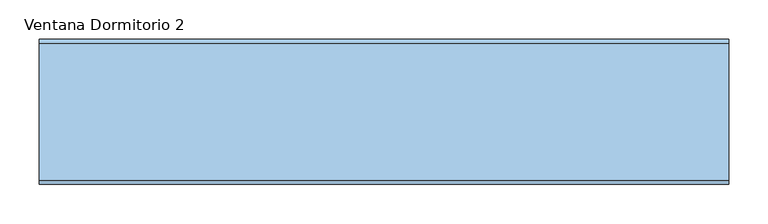
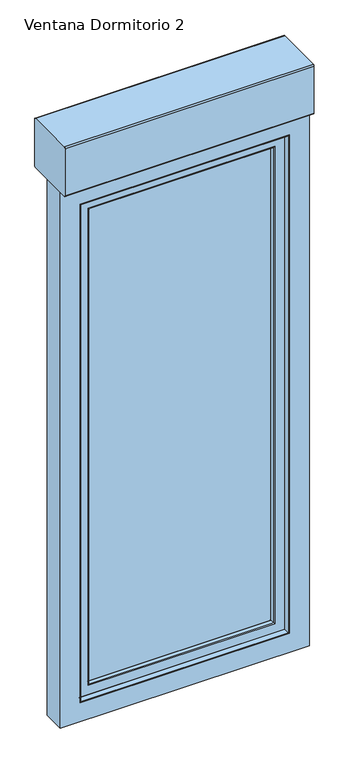
"""IFC4 building model written with IfcOpenShell, lengths in millimetres: window geometry, 2019_ES_Ventana_Replus_re80pvc301_10100_box_1-Hoja_con-Compacto : Ventana Dormitorio 2."""

from ifc_helpers import new_model, si_unit, point, frame, frame_2d, origin, place, context, project, spatial, polyline, circle_curve, ellipse_curve, trimmed, segment, composite_curve, outline, extrude, source, transform, mapped, element, save
from ifc_brep_helpers import plane_surface, cylinder_surface, advanced_brep


def ventana_dormitorio_2_c32e29da(model_context):
    return source(origin(), model_context, "Body", "SolidModel", [
        extrude(outline(composite_curve([segment(trimmed(circle_curve(frame_2d((-55.0, 2815.0)), 5.0), [point((-55.0, 2810.0))], [point((-60.0, 2815.0))], False, "CARTESIAN"), True, "CONTINUOUS"), segment(polyline([(-60.0, 2815.0), (-60.0, 2990.0)]), True, "CONTINUOUS"), segment(trimmed(circle_curve(frame_2d((-55.0, 2990.0)), 5.0), [point((-60.0, 2990.0))], [point((-55.0, 2995.0))], False, "CARTESIAN"), True, "CONTINUOUS"), segment(polyline([(-55.0, 2995.0), (120.0, 2995.0)]), True, "CONTINUOUS"), segment(trimmed(circle_curve(frame_2d((120.0, 2990.0)), 5.0), [point((120.0, 2995.0))], [point((125.0, 2990.0))], False, "CARTESIAN"), True, "CONTINUOUS"), segment(polyline([(125.0, 2990.0), (125.0, 2815.0)]), True, "CONTINUOUS"), segment(trimmed(circle_curve(frame_2d((120.0, 2815.0)), 5.0), [point((125.0, 2815.0))], [point((120.0, 2810.0))], False, "CARTESIAN"), True, "CONTINUOUS"), segment(polyline([(120.0, 2810.0), (-55.0, 2810.0)]), True, "CONTINUOUS")], self_intersect=False)), frame((-440.0, 0.0, 0.0), z_axis=(1.0, 0.0, 0.0), x_axis=(0.0, 1.0, 0.0)), (0.0, 0.0, 1.0), 880.0),
        extrude(outline(polyline([(78.4999991, 1470.0), (118.4999991, 1470.0), (118.4999991, 1360.0), (98.4999991, 1360.0), (98.4999991, 1450.0), (78.4999991, 1450.0), (78.4999991, 1470.0)])), frame((-374.1999993, 0.0, 0.0), z_axis=(1.0, 0.0, 0.0), x_axis=(0.0, 1.0, 0.0)), (0.0, 0.0, 1.0), 12.0),
        extrude(outline(polyline([(-353.9687607, 78.4999991), (-353.9687607, 68.4999991), (-382.4312378, 68.4999991), (-382.4312378, 78.4999991), (-353.9687607, 78.4999991)])), frame((0.0, 0.0, 1435.217127), z_axis=(0.0, 0.0, 1.0), x_axis=(1.0, 0.0, 0.0)), (0.0, 0.0, 1.0), 49.565746),
        extrude(outline(polyline([(909.8, 337.1999993), (2707.2, 337.1999993), (2707.2, -337.1999993), (909.8, -337.1999993), (909.8, 337.1999993)]), holes=[polyline([(2699.2, 329.1999993), (917.8, 329.1999993), (917.8, -329.1999993), (2699.2, -329.1999993), (2699.2, 329.1999993)])]), frame((0.0, 10.9999999, 0.0), z_axis=(0.0, 1.0, 0.0), x_axis=(0.0, 0.0, 1.0)), (0.0, 0.0, 1.0), 16.0),
        extrude(outline(polyline([(909.8131934, 337.1868058), (2707.1868066, 337.1868058), (2707.1868066, -337.1868058), (909.8131934, -337.1868058), (909.8131934, 337.1868058)]), holes=[polyline([(2699.2, 329.1999993), (917.8, 329.1999993), (917.8, -329.1999993), (2699.2, -329.1999993), (2699.2, 329.1999993)])]), frame((0.0, 31.0000001, 0.0), z_axis=(0.0, 1.0, 0.0), x_axis=(0.0, 0.0, 1.0)), (0.0, 0.0, 1.0), 16.0),
        extrude(outline(polyline([(337.1999993, 6.9999997), (-337.1999993, 6.9999997), (-337.1999993, 10.9999999), (337.1999993, 10.9999999), (337.1999993, 6.9999997)])), frame((0.0, 0.0, 903.7946451), z_axis=(0.0, 0.0, 1.0), x_axis=(1.0, 0.0, 0.0)), (0.0, 0.0, 1.0), 1809.4053549),
        extrude(outline(polyline([(337.1999993, 26.9999999), (-337.1999993, 26.9999999), (-337.1999993, 31.0000001), (337.1999993, 31.0000001), (337.1999993, 26.9999999)])), frame((0.0, 0.0, 903.7946451), z_axis=(0.0, 0.0, 1.0), x_axis=(1.0, 0.0, 0.0)), (0.0, 0.0, 1.0), 1809.4053549),
        extrude(outline(polyline([(337.1999993, 47.0000001), (-337.1999993, 47.0000001), (-337.1999993, 51.0000003), (337.1999993, 51.0000003), (337.1999993, 47.0000001)])), frame((0.0, 0.0, 903.7946451), z_axis=(0.0, 0.0, 1.0), x_axis=(1.0, 0.0, 0.0)), (0.0, 0.0, 1.0), 1809.4053549),
        advanced_brep(
        [(327.2913171, -9.2764571, 2697.2913178), (327.2913171, -9.2764571, 922.7086822), (330.1890946, -11.5, 919.8109047), (330.1890946, -11.5, 2700.1890953), (370.1999993, -11.5, 879.8), (370.1999993, -11.5, 2740.2), (-370.1999993, -11.5, 2740.2), (-370.1999993, -11.5, 879.8), (-330.1890946, -11.5, 919.8109047), (-330.1890946, -11.5, 2700.1890953), (-327.2913171, -9.2764571, 922.7086822), (324.1757968, 2.3508228, 2694.1757976), (324.1757968, 2.3508228, 925.8242024), (-324.1757968, 2.3508228, 925.8242024), (324.6739305, 3.0000033, 2694.6739313), (324.6739305, 3.0000033, 925.3260687), (-324.6739305, 3.0000033, 925.3260687), (331.1999993, 3.0000033, 2701.2), (331.1999993, 3.0000033, 918.8), (-331.1999993, 3.0000033, 918.8), (-331.1999993, 3.0000033, 2701.2), (-324.6739305, 3.0000033, 2694.6739313), (331.1999993, 6.9999997, 2701.2), (331.1999993, 6.9999997, 918.8), (-331.1999993, 6.9999997, 918.8), (351.8162192, 6.9999997, 2721.8162199), (351.8162192, 6.9999997, 898.1837801), (-351.8162192, 6.9999997, 898.1837801), (-351.8162192, 6.9999997, 2721.8162199), (-331.1999993, 6.9999997, 2701.2), (349.1999993, 25.6153717, 2719.2), (349.1999993, 25.6153717, 900.8), (-349.1999993, 25.6153717, 900.8), (349.1999993, 56.4999995, 2719.2), (349.1999993, 56.4999995, 900.8), (-349.1999993, 56.4999995, 900.8), (-349.1999993, 56.4999995, 2719.2), (337.1999993, 56.4999995, 2707.2), (337.1999993, 56.4999995, 912.8), (-337.1999993, 56.4999995, 912.8), (-337.1999993, 56.4999995, 2707.2), (337.1999993, 51.0000003, 2707.2), (337.1999993, 51.0000003, 912.8), (-337.1999993, 51.0000003, 912.8), (-337.1999993, 51.0000003, 2707.2), (326.007687, 51.0000003, 2696.0076877), (326.007687, 51.0000003, 923.9923123), (-326.007687, 51.0000003, 923.9923123), (-326.007687, 51.0000003, 2696.0076877), (325.4940999, 51.6693201, 2695.4941006), (325.4940999, 51.6693201, 924.5058994), (-325.4940999, 51.6693201, 924.5058994), (328.8993918, 64.3780426, 2698.8993925), (328.8993918, 64.3780426, 921.1006075), (-328.8993918, 64.3780426, 921.1006075), (332.6234971, 67.3403297, 2702.6234978), (332.6234971, 67.3403297, 917.3765022), (-332.6234971, 67.3403297, 917.3765022), (345.6488427, 67.7951848, 2715.6488434), (345.6488427, 67.7951848, 904.3511566), (-345.6488427, 67.7951848, 904.3511566), (346.1999993, 67.2629391, 2716.2), (346.1999993, 67.2629391, 903.8), (-346.1999993, 67.2629391, 903.8), (347.4370593, 68.4999991, 2717.43706), (347.4370593, 68.4999991, 902.56294), (-347.4370593, 68.4999991, 902.56294), (400.1999993, 68.4999991, 2770.2), (400.1999993, 68.4999991, 849.8), (-400.1999993, 68.4999991, 849.8), (-400.1999993, 68.4999991, 2770.2), (-347.4370593, 68.4999991, 2717.43706), (403.1999993, 65.4999991, 2773.2), (403.1999993, 65.4999991, 846.8), (-403.1999993, 65.4999991, 846.8), (403.1999993, 50.0, 2773.2), (403.1999993, 50.0, 846.8), (-403.1999993, 50.0, 846.8), (-403.1999993, 50.0, 2773.2), (383.1999993, 50.0, 2753.2), (383.1999993, 50.0, 866.8), (-383.1999993, 50.0, 866.8), (-383.1999993, 50.0, 2753.2), (383.1999993, 11.9999991, 2753.2), (383.1999993, 11.9999991, 866.8), (-383.1999993, 11.9999991, 866.8), (-383.1999993, 11.9999991, 2753.2), (370.1999993, 11.9999991, 2740.2), (370.1999993, 11.9999991, 879.8), (-370.1999993, 11.9999991, 879.8), (-370.1999993, 11.9999991, 2740.2), (-327.2913171, -9.2764571, 2697.2913178), (-324.1757968, 2.3508228, 2694.1757976), (-349.1999993, 25.6153717, 2719.2), (-325.4940999, 51.6693201, 2695.4941006), (-328.8993918, 64.3780426, 2698.8993925), (-332.6234971, 67.3403297, 2702.6234978), (-345.6488427, 67.7951848, 2715.6488434), (-346.1999993, 67.2629391, 2716.2), (-403.1999993, 65.4999991, 2773.2)],
        [
            (0, 1),
            (1, 2, ellipse_curve(frame((330.1890946, -8.5, 919.8109047), z_axis=(0.7071067811865475, 0.0, 0.7071067811865475), x_axis=(-0.7071067811865474, 0.0, 0.7071067811865476)), 4.2426407, 3.0)),
            (2, 3),
            (3, 0, ellipse_curve(frame((330.1890946, -8.5, 2700.1890953), z_axis=(0.7071067811865475, 0.0, -0.7071067811865475), x_axis=(0.7071067811865474, 0.0, 0.7071067811865476)), 4.2426407, 3.0)),
            (4, 5),
            (5, 6),
            (6, 7),
            (7, 4),
            (2, 8),
            (8, 9),
            (9, 3),
            (1, 10),
            (10, 8, ellipse_curve(frame((-330.1890946, -8.5, 919.8109047), z_axis=(0.7071067811865475, 0.0, -0.7071067811865475), x_axis=(0.7071067811865476, 0.0, 0.7071067811865474)), 4.2426407, 3.0)),
            (11, 12),
            (12, 1),
            (0, 11),
            (12, 13),
            (13, 10),
            (14, 15),
            (15, 12, ellipse_curve(frame((324.6739305, 2.4842973, 925.3260687), z_axis=(0.7071067811865475, 0.0, 0.7071067811865475), x_axis=(-0.7071067811865474, 0.0, 0.7071067811865476)), 0.7293184, 0.515706)),
            (11, 14, ellipse_curve(frame((324.6739305, 2.4842973, 2694.6739313), z_axis=(0.7071067811865475, 0.0, -0.7071067811865475), x_axis=(0.7071067811865474, 0.0, 0.7071067811865476)), 0.7293184, 0.515706)),
            (15, 16),
            (16, 13, ellipse_curve(frame((-324.6739305, 2.4842973, 925.3260687), z_axis=(0.7071067811865475, 0.0, -0.7071067811865475), x_axis=(0.7071067811865476, 0.0, 0.7071067811865474)), 0.7293184, 0.515706)),
            (17, 18),
            (18, 19),
            (19, 20),
            (20, 17),
            (14, 21),
            (21, 16),
            (22, 23),
            (23, 18),
            (17, 22),
            (23, 24),
            (24, 19),
            (25, 26),
            (26, 27),
            (27, 28),
            (28, 25),
            (22, 29),
            (29, 24),
            (30, 31),
            (31, 26),
            (25, 30),
            (31, 32),
            (32, 27),
            (33, 34),
            (34, 31),
            (30, 33),
            (34, 35),
            (35, 32),
            (33, 36),
            (36, 35),
            (37, 38),
            (38, 39),
            (39, 40),
            (40, 37),
            (41, 42),
            (42, 38),
            (37, 41),
            (42, 43),
            (43, 39),
            (41, 44),
            (44, 43),
            (45, 46),
            (46, 47),
            (47, 48),
            (48, 45),
            (49, 50),
            (50, 46, ellipse_curve(frame((326.007687, 51.5317048, 923.9923123), z_axis=(0.7071067811865475, 0.0, 0.7071067811865475), x_axis=(-0.7071067811865474, 0.0, 0.7071067811865476)), 0.7519437, 0.5317045)),
            (45, 49, ellipse_curve(frame((326.007687, 51.5317048, 2696.0076877), z_axis=(0.7071067811865475, 0.0, -0.7071067811865475), x_axis=(0.7071067811865474, 0.0, 0.7071067811865476)), 0.7519437, 0.5317045)),
            (50, 51),
            (51, 47, ellipse_curve(frame((-326.007687, 51.5317048, 923.9923123), z_axis=(0.7071067811865475, 0.0, -0.7071067811865475), x_axis=(0.7071067811865476, 0.0, 0.7071067811865474)), 0.7519437, 0.5317045)),
            (52, 53),
            (53, 50),
            (49, 52),
            (53, 54),
            (54, 51),
            (55, 56),
            (56, 53, ellipse_curve(frame((332.7630951, 63.3427664, 917.2369042), z_axis=(0.7071067811865475, 0.0, 0.7071067811865475), x_axis=(-0.7071067811865474, 0.0, 0.7071067811865476)), 5.6568542, 4.0)),
            (52, 55, ellipse_curve(frame((332.7630951, 63.3427664, 2702.7630958), z_axis=(0.7071067811865475, 0.0, -0.7071067811865475), x_axis=(0.7071067811865474, 0.0, 0.7071067811865476)), 5.6568542, 4.0)),
            (56, 57),
            (57, 54, ellipse_curve(frame((-332.7630951, 63.3427664, 917.2369042), z_axis=(0.7071067811865475, 0.0, -0.7071067811865475), x_axis=(0.7071067811865476, 0.0, 0.7071067811865474)), 5.6568542, 4.0)),
            (58, 59),
            (59, 56),
            (55, 58),
            (59, 60),
            (60, 57),
            (61, 62),
            (62, 59, ellipse_curve(frame((345.6674291, 67.2629391, 904.3325701), z_axis=(0.7071067811865475, 0.0, 0.7071067811865475), x_axis=(-0.7071067811865474, 0.0, 0.7071067811865476)), 0.7531679, 0.5325701)),
            (58, 61, ellipse_curve(frame((345.6674291, 67.2629391, 2715.6674299), z_axis=(0.7071067811865475, 0.0, -0.7071067811865475), x_axis=(0.7071067811865474, 0.0, 0.7071067811865476)), 0.7531679, 0.5325701)),
            (62, 63),
            (63, 60, ellipse_curve(frame((-345.6674291, 67.2629391, 904.3325701), z_axis=(0.7071067811865475, 0.0, -0.7071067811865475), x_axis=(0.7071067811865476, 0.0, 0.7071067811865474)), 0.7531679, 0.5325701)),
            (64, 65),
            (65, 62, ellipse_curve(frame((347.4370593, 67.2629391, 902.56294), z_axis=(0.7071067811865475, 0.0, 0.7071067811865475), x_axis=(-0.7071067811865474, 0.0, 0.7071067811865476)), 1.7494671, 1.23706)),
            (61, 64, ellipse_curve(frame((347.4370593, 67.2629391, 2717.43706), z_axis=(0.7071067811865475, 0.0, -0.7071067811865475), x_axis=(0.7071067811865474, 0.0, 0.7071067811865476)), 1.7494671, 1.23706)),
            (65, 66),
            (66, 63, ellipse_curve(frame((-347.4370593, 67.2629391, 902.56294), z_axis=(0.7071067811865475, 0.0, -0.7071067811865475), x_axis=(0.7071067811865476, 0.0, 0.7071067811865474)), 1.7494671, 1.23706)),
            (67, 68),
            (68, 69),
            (69, 70),
            (70, 67),
            (64, 71),
            (71, 66),
            (72, 73),
            (73, 68, ellipse_curve(frame((400.1999993, 65.4999991, 849.8), z_axis=(0.7071067811865475, 0.0, 0.7071067811865475), x_axis=(-0.7071067811865474, 0.0, 0.7071067811865476)), 4.2426407, 3.0)),
            (67, 72, ellipse_curve(frame((400.1999993, 65.4999991, 2770.2), z_axis=(0.7071067811865475, 0.0, -0.7071067811865475), x_axis=(0.7071067811865474, 0.0, 0.7071067811865476)), 4.2426407, 3.0)),
            (73, 74),
            (74, 69, ellipse_curve(frame((-400.1999993, 65.4999991, 849.8), z_axis=(0.7071067811865475, 0.0, -0.7071067811865475), x_axis=(0.7071067811865476, 0.0, 0.7071067811865474)), 4.2426407, 3.0)),
            (75, 76),
            (76, 73),
            (72, 75),
            (76, 77),
            (77, 74),
            (75, 78),
            (78, 77),
            (79, 80),
            (80, 81),
            (81, 82),
            (82, 79),
            (79, 83),
            (83, 84),
            (84, 80),
            (84, 85),
            (85, 81),
            (83, 86),
            (86, 85),
            (87, 88),
            (88, 89),
            (89, 90),
            (90, 87),
            (87, 5),
            (4, 88),
            (7, 89),
            (10, 91),
            (91, 9, ellipse_curve(frame((-330.1890946, -8.5, 2700.1890953), z_axis=(-0.7071067811865475, 0.0, -0.7071067811865475), x_axis=(0.7071067811865474, 0.0, -0.7071067811865476)), 4.2426407, 3.0)),
            (13, 92),
            (92, 91),
            (21, 92, ellipse_curve(frame((-324.6739305, 2.4842973, 2694.6739313), z_axis=(-0.7071067811865475, 0.0, -0.7071067811865475), x_axis=(0.7071067811865474, 0.0, -0.7071067811865476)), 0.7293184, 0.515706)),
            (29, 20),
            (32, 93),
            (93, 28),
            (36, 93),
            (44, 40),
            (51, 94),
            (94, 48, ellipse_curve(frame((-326.007687, 51.5317048, 2696.0076877), z_axis=(-0.7071067811865475, 0.0, -0.7071067811865475), x_axis=(0.7071067811865474, 0.0, -0.7071067811865476)), 0.7519437, 0.5317045)),
            (54, 95),
            (95, 94),
            (57, 96),
            (96, 95, ellipse_curve(frame((-332.7630951, 63.3427664, 2702.7630958), z_axis=(-0.7071067811865475, 0.0, -0.7071067811865475), x_axis=(0.7071067811865474, 0.0, -0.7071067811865476)), 5.6568542, 4.0)),
            (60, 97),
            (97, 96),
            (63, 98),
            (98, 97, ellipse_curve(frame((-345.6674291, 67.2629391, 2715.6674299), z_axis=(-0.7071067811865475, 0.0, -0.7071067811865475), x_axis=(0.7071067811865474, 0.0, -0.7071067811865476)), 0.7531679, 0.5325701)),
            (71, 98, ellipse_curve(frame((-347.4370593, 67.2629391, 2717.43706), z_axis=(-0.7071067811865475, 0.0, -0.7071067811865475), x_axis=(0.7071067811865474, 0.0, -0.7071067811865476)), 1.7494671, 1.23706)),
            (74, 99),
            (99, 70, ellipse_curve(frame((-400.1999993, 65.4999991, 2770.2), z_axis=(-0.7071067811865475, 0.0, -0.7071067811865475), x_axis=(0.7071067811865474, 0.0, -0.7071067811865476)), 4.2426407, 3.0)),
            (78, 99),
            (86, 82),
            (6, 90),
            (91, 0),
            (92, 11),
            (93, 30),
            (94, 49),
            (95, 52),
            (96, 55),
            (97, 58),
            (98, 61),
            (99, 72),
        ],
        [
            cylinder_surface(frame((330.1890946, -8.5, 2773.2), z_axis=(0.0, 0.0, 1.0), x_axis=(-1.0, 0.0, 0.0)), 3.0),
            plane_surface(frame((-370.1999993, -11.5, 2740.2), z_axis=(0.0, -1.0, 0.0), x_axis=(1.0, 0.0, 0.0))),
            cylinder_surface(frame((403.1999993, -8.5, 919.8109047), z_axis=(1.0, 0.0, 0.0), x_axis=(0.0, 0.0, 1.0)), 3.0),
            plane_surface(frame((327.2913171, -9.2764571, 2697.2913178), z_axis=(-0.9659258263570549, -0.25881904484879154, 0.0), x_axis=(0.0, 0.0, -1.0))),
            plane_surface(frame((327.2913171, -9.2764571, 922.7086822), z_axis=(0.0, -0.2588190448487884, 0.9659258263570558), x_axis=(-1.0, 0.0, 0.0))),
            cylinder_surface(frame((324.6739305, 2.4842973, 2773.2), z_axis=(0.0, 0.0, 1.0), x_axis=(-1.0, 0.0, 0.0)), 0.515706),
            cylinder_surface(frame((403.1999993, 2.4842973, 925.3260687), z_axis=(1.0, 0.0, 0.0), x_axis=(0.0, 0.0, 1.0)), 0.515706),
            plane_surface(frame((-324.6739305, 3.0000033, 2694.6739313), z_axis=(0.0, 1.0, 0.0), x_axis=(1.0, 0.0, 0.0))),
            plane_surface(frame((331.1999993, 3.0000033, 2701.2), z_axis=(-1.0, 0.0, 0.0), x_axis=(0.0, 0.0, -1.0))),
            plane_surface(frame((331.1999993, 3.0000033, 918.8), z_axis=(0.0, 0.0, 1.0), x_axis=(-1.0, 0.0, 0.0))),
            plane_surface(frame((-331.1999993, 6.9999997, 2701.2), z_axis=(0.0, 1.0, 0.0), x_axis=(1.0, 0.0, 0.0))),
            plane_surface(frame((351.8162192, 6.9999997, 2721.8162199), z_axis=(-0.9902680687415736, -0.13917310096004265, 0.0), x_axis=(0.0, 0.0, -1.0))),
            plane_surface(frame((351.8162192, 6.9999997, 898.1837801), z_axis=(0.0, -0.13917310096003946, 0.990268068741574), x_axis=(-1.0, 0.0, 0.0))),
            plane_surface(frame((349.1999993, 25.6153717, 2719.2), z_axis=(-1.0, 0.0, 0.0), x_axis=(0.0, 0.0, -1.0))),
            plane_surface(frame((349.1999993, 25.6153717, 900.8), z_axis=(0.0, 0.0, 1.0), x_axis=(-1.0, 0.0, 0.0))),
            plane_surface(frame((-349.1999993, 56.4999995, 2719.2), z_axis=(0.0, -1.0, 0.0), x_axis=(1.0, 0.0, 0.0))),
            plane_surface(frame((337.1999993, 56.4999995, 2707.2), z_axis=(1.0, 0.0, 0.0), x_axis=(0.0, 0.0, -1.0))),
            plane_surface(frame((337.1999993, 56.4999995, 912.8), z_axis=(0.0, 0.0, -1.0), x_axis=(-1.0, 0.0, 0.0))),
            plane_surface(frame((-337.1999993, 51.0000003, 2707.2), z_axis=(0.0, -1.0, 0.0), x_axis=(1.0, 0.0, 0.0))),
            cylinder_surface(frame((326.007687, 51.5317048, 2773.2), z_axis=(0.0, 0.0, 1.0), x_axis=(-1.0, 0.0, 0.0)), 0.5317045),
            cylinder_surface(frame((403.1999993, 51.5317048, 923.9923123), z_axis=(1.0, 0.0, 0.0), x_axis=(0.0, 0.0, 1.0)), 0.5317045),
            plane_surface(frame((325.4940999, 51.6693201, 2695.4941006), z_axis=(-0.9659258262890665, 0.2588190451025274, 0.0), x_axis=(0.0, 0.0, -1.0))),
            plane_surface(frame((325.4940999, 51.6693201, 924.5058994), z_axis=(0.0, 0.25881904510253056, 0.9659258262890658), x_axis=(-1.0, 0.0, 0.0))),
            cylinder_surface(frame((332.7630951, 63.3427664, 2773.2), z_axis=(0.0, 0.0, 1.0), x_axis=(-1.0, 0.0, 0.0)), 4.0),
            cylinder_surface(frame((403.1999993, 63.3427664, 917.2369042), z_axis=(1.0, 0.0, 0.0), x_axis=(0.0, 0.0, 1.0)), 4.0),
            plane_surface(frame((332.6234971, 67.3403297, 2702.6234978), z_axis=(-0.034899496702507804, 0.9993908270190955, 0.0), x_axis=(0.0, 0.0, -1.0))),
            plane_surface(frame((332.6234971, 67.3403297, 917.3765022), z_axis=(0.0, 0.9993908270190957, 0.03489949670250458), x_axis=(-1.0, 0.0, 0.0))),
            cylinder_surface(frame((345.6674291, 67.2629391, 2773.2), z_axis=(0.0, 0.0, 1.0), x_axis=(-1.0, 0.0, 0.0)), 0.5325701),
            cylinder_surface(frame((403.1999993, 67.2629391, 904.3325701), z_axis=(1.0, 0.0, 0.0), x_axis=(0.0, 0.0, 1.0)), 0.5325701),
            cylinder_surface(frame((347.4370593, 67.2629391, 2773.2), z_axis=(0.0, 0.0, 1.0), x_axis=(-1.0, 0.0, 0.0)), 1.23706),
            cylinder_surface(frame((403.1999993, 67.2629391, 902.56294), z_axis=(1.0, 0.0, 0.0), x_axis=(0.0, 0.0, 1.0)), 1.23706),
            plane_surface(frame((-347.4370593, 68.4999991, 2717.43706), z_axis=(0.0, 1.0, 0.0), x_axis=(1.0, 0.0, 0.0))),
            cylinder_surface(frame((400.1999993, 65.4999991, 2773.2), z_axis=(0.0, 0.0, 1.0), x_axis=(-1.0, 0.0, 0.0)), 3.0),
            cylinder_surface(frame((403.1999993, 65.4999991, 849.8), z_axis=(1.0, 0.0, 0.0), x_axis=(0.0, 0.0, 1.0)), 3.0),
            plane_surface(frame((403.1999993, 65.4999991, 2773.2), z_axis=(1.0, 0.0, 0.0), x_axis=(0.0, 0.0, -1.0))),
            plane_surface(frame((403.1999993, 65.4999991, 846.8), z_axis=(0.0, 0.0, -1.0), x_axis=(-1.0, 0.0, 0.0))),
            plane_surface(frame((-399.2000019, 50.0, 2769.2000027), z_axis=(0.0, -1.0, 0.0), x_axis=(1.0, 0.0, 0.0))),
            plane_surface(frame((383.1999993, 45.0999991, 2753.2), z_axis=(1.0, 0.0, 0.0), x_axis=(0.0, 0.0, -1.0))),
            plane_surface(frame((383.1999993, 45.0999991, 866.8), z_axis=(0.0, 0.0, -1.0), x_axis=(-1.0, 0.0, 0.0))),
            plane_surface(frame((-375.7000002, 11.9999991, 2745.7000009), z_axis=(0.0, -1.0, 0.0), x_axis=(1.0, 0.0, 0.0))),
            plane_surface(frame((370.1999993, 1.4999991, 2740.2), z_axis=(1.0, 0.0, 0.0), x_axis=(0.0, 0.0, -1.0))),
            plane_surface(frame((370.1999993, 1.4999991, 879.8), z_axis=(0.0, 0.0, -1.0), x_axis=(-1.0, 0.0, 0.0))),
            cylinder_surface(frame((-330.1890946, -8.5, 846.8), z_axis=(0.0, 0.0, -1.0), x_axis=(1.0, 0.0, 0.0)), 3.0),
            plane_surface(frame((-327.2913171, -9.2764571, 922.7086822), z_axis=(0.9659258263570565, -0.25881904484878526, 0.0), x_axis=(0.0, 0.0, 1.0))),
            cylinder_surface(frame((-324.6739305, 2.4842973, 846.8), z_axis=(0.0, 0.0, -1.0), x_axis=(1.0, 0.0, 0.0)), 0.515706),
            plane_surface(frame((-331.1999993, 3.0000033, 918.8), z_axis=(1.0, 0.0, 0.0), x_axis=(0.0, 0.0, 1.0))),
            plane_surface(frame((-351.8162192, 6.9999997, 898.1837801), z_axis=(0.9902680687415745, -0.13917310096003627, 0.0), x_axis=(0.0, 0.0, 1.0))),
            plane_surface(frame((-349.1999993, 25.6153717, 900.8), z_axis=(1.0, 0.0, 0.0), x_axis=(0.0, 0.0, 1.0))),
            plane_surface(frame((-337.1999993, 56.4999995, 912.8), z_axis=(-1.0, 0.0, 0.0), x_axis=(0.0, 0.0, 1.0))),
            cylinder_surface(frame((-326.007687, 51.5317048, 846.8), z_axis=(0.0, 0.0, -1.0), x_axis=(1.0, 0.0, 0.0)), 0.5317045),
            plane_surface(frame((-325.4940999, 51.6693201, 924.5058994), z_axis=(0.9659258262890649, 0.2588190451025337, 0.0), x_axis=(0.0, 0.0, 1.0))),
            cylinder_surface(frame((-332.7630951, 63.3427664, 846.8), z_axis=(0.0, 0.0, -1.0), x_axis=(1.0, 0.0, 0.0)), 4.0),
            plane_surface(frame((-332.6234971, 67.3403297, 917.3765022), z_axis=(0.03489949670250135, 0.9993908270190958, 0.0), x_axis=(0.0, 0.0, 1.0))),
            cylinder_surface(frame((-345.6674291, 67.2629391, 846.8), z_axis=(0.0, 0.0, -1.0), x_axis=(1.0, 0.0, 0.0)), 0.5325701),
            cylinder_surface(frame((-347.4370593, 67.2629391, 846.8), z_axis=(0.0, 0.0, -1.0), x_axis=(1.0, 0.0, 0.0)), 1.23706),
            cylinder_surface(frame((-400.1999993, 65.4999991, 846.8), z_axis=(0.0, 0.0, -1.0), x_axis=(1.0, 0.0, 0.0)), 3.0),
            plane_surface(frame((-403.1999993, 65.4999991, 846.8), z_axis=(-1.0, 0.0, 0.0), x_axis=(0.0, 0.0, 1.0))),
            plane_surface(frame((-383.1999993, 45.0999991, 866.8), z_axis=(-1.0, 0.0, 0.0), x_axis=(0.0, 0.0, 1.0))),
            plane_surface(frame((-370.1999993, 1.4999991, 879.8), z_axis=(-1.0, 0.0, 0.0), x_axis=(0.0, 0.0, 1.0))),
            cylinder_surface(frame((-403.1999993, -8.5, 2700.1890953), z_axis=(-1.0, 0.0, 0.0), x_axis=(0.0, 0.0, -1.0)), 3.0),
            plane_surface(frame((-327.2913171, -9.2764571, 2697.2913178), z_axis=(0.0, -0.2588190448487884, -0.9659258263570557), x_axis=(1.0, 0.0, 0.0))),
            cylinder_surface(frame((-403.1999993, 2.4842973, 2694.6739313), z_axis=(-1.0, 0.0, 0.0), x_axis=(0.0, 0.0, -1.0)), 0.515706),
            plane_surface(frame((-331.1999993, 3.0000033, 2701.2), z_axis=(0.0, 0.0, -1.0), x_axis=(1.0, 0.0, 0.0))),
            plane_surface(frame((-351.8162192, 6.9999997, 2721.8162199), z_axis=(0.0, -0.13917310096003946, -0.990268068741574), x_axis=(1.0, 0.0, 0.0))),
            plane_surface(frame((-349.1999993, 25.6153717, 2719.2), z_axis=(0.0, 0.0, -1.0), x_axis=(1.0, 0.0, 0.0))),
            plane_surface(frame((-337.1999993, 56.4999995, 2707.2), z_axis=(0.0, 0.0, 1.0), x_axis=(1.0, 0.0, 0.0))),
            cylinder_surface(frame((-403.1999993, 51.5317048, 2696.0076877), z_axis=(-1.0, 0.0, 0.0), x_axis=(0.0, 0.0, -1.0)), 0.5317045),
            plane_surface(frame((-325.4940999, 51.6693201, 2695.4941006), z_axis=(0.0, 0.25881904510253056, -0.9659258262890658), x_axis=(1.0, 0.0, 0.0))),
            cylinder_surface(frame((-403.1999993, 63.3427664, 2702.7630958), z_axis=(-1.0, 0.0, 0.0), x_axis=(0.0, 0.0, -1.0)), 4.0),
            plane_surface(frame((-332.6234971, 67.3403297, 2702.6234978), z_axis=(0.0, 0.9993908270190957, -0.03489949670250458), x_axis=(1.0, 0.0, 0.0))),
            cylinder_surface(frame((-403.1999993, 67.2629391, 2715.6674299), z_axis=(-1.0, 0.0, 0.0), x_axis=(0.0, 0.0, -1.0)), 0.5325701),
            cylinder_surface(frame((-403.1999993, 67.2629391, 2717.43706), z_axis=(-1.0, 0.0, 0.0), x_axis=(0.0, 0.0, -1.0)), 1.23706),
            cylinder_surface(frame((-403.1999993, 65.4999991, 2770.2), z_axis=(-1.0, 0.0, 0.0), x_axis=(0.0, 0.0, -1.0)), 3.0),
            plane_surface(frame((-403.1999993, 65.4999991, 2773.2), z_axis=(0.0, 0.0, 1.0), x_axis=(1.0, 0.0, 0.0))),
            plane_surface(frame((-383.1999993, 45.0999991, 2753.2), z_axis=(0.0, 0.0, 1.0), x_axis=(1.0, 0.0, 0.0))),
            plane_surface(frame((-370.1999993, 1.4999991, 2740.2), z_axis=(0.0, 0.0, 1.0), x_axis=(1.0, 0.0, 0.0))),
        ],
        [
            (0, [[1, 2, 3, 4]]),
            (1, [[5, 6, 7, 8], [-3, 9, 10, 11]]),
            (2, [[12, 13, -9, -2]]),
            (3, [[14, 15, -1, 16]]),
            (4, [[17, 18, -12, -15]]),
            (5, [[19, 20, -14, 21]]),
            (6, [[22, 23, -17, -20]]),
            (7, [[24, 25, 26, 27], [-19, 28, 29, -22]]),
            (8, [[30, 31, -24, 32]]),
            (9, [[33, 34, -25, -31]]),
            (10, [[35, 36, 37, 38], [-30, 39, 40, -33]]),
            (11, [[41, 42, -35, 43]]),
            (12, [[44, 45, -36, -42]]),
            (13, [[46, 47, -41, 48]]),
            (14, [[49, 50, -44, -47]]),
            (15, [[-46, 51, 52, -49], [53, 54, 55, 56]]),
            (16, [[57, 58, -53, 59]]),
            (17, [[60, 61, -54, -58]]),
            (18, [[-57, 62, 63, -60], [64, 65, 66, 67]]),
            (19, [[68, 69, -64, 70]]),
            (20, [[71, 72, -65, -69]]),
            (21, [[73, 74, -68, 75]]),
            (22, [[76, 77, -71, -74]]),
            (23, [[78, 79, -73, 80]]),
            (24, [[81, 82, -76, -79]]),
            (25, [[83, 84, -78, 85]]),
            (26, [[86, 87, -81, -84]]),
            (27, [[88, 89, -83, 90]]),
            (28, [[91, 92, -86, -89]]),
            (29, [[93, 94, -88, 95]]),
            (30, [[96, 97, -91, -94]]),
            (31, [[98, 99, 100, 101], [-93, 102, 103, -96]]),
            (32, [[104, 105, -98, 106]]),
            (33, [[107, 108, -99, -105]]),
            (34, [[109, 110, -104, 111]]),
            (35, [[112, 113, -107, -110]]),
            (36, [[-109, 114, 115, -112], [116, 117, 118, 119]]),
            (37, [[120, 121, 122, -116]]),
            (38, [[123, 124, -117, -122]]),
            (39, [[-121, 125, 126, -123], [127, 128, 129, 130]]),
            (40, [[131, -5, 132, -127]]),
            (41, [[-8, 133, -128, -132]]),
            (42, [[134, 135, -10, -13]]),
            (43, [[136, 137, -134, -18]]),
            (44, [[-29, 138, -136, -23]]),
            (45, [[-40, 139, -26, -34]]),
            (46, [[140, 141, -37, -45]]),
            (47, [[-52, 142, -140, -50]]),
            (48, [[-63, 143, -55, -61]]),
            (49, [[144, 145, -66, -72]]),
            (50, [[146, 147, -144, -77]]),
            (51, [[148, 149, -146, -82]]),
            (52, [[150, 151, -148, -87]]),
            (53, [[152, 153, -150, -92]]),
            (54, [[-103, 154, -152, -97]]),
            (55, [[155, 156, -100, -108]]),
            (56, [[-115, 157, -155, -113]]),
            (57, [[-126, 158, -118, -124]]),
            (58, [[-7, 159, -129, -133]]),
            (59, [[160, -4, -11, -135]]),
            (60, [[161, -16, -160, -137]]),
            (61, [[-28, -21, -161, -138]]),
            (62, [[-39, -32, -27, -139]]),
            (63, [[162, -43, -38, -141]]),
            (64, [[-51, -48, -162, -142]]),
            (65, [[-62, -59, -56, -143]]),
            (66, [[163, -70, -67, -145]]),
            (67, [[164, -75, -163, -147]]),
            (68, [[165, -80, -164, -149]]),
            (69, [[166, -85, -165, -151]]),
            (70, [[167, -90, -166, -153]]),
            (71, [[-102, -95, -167, -154]]),
            (72, [[168, -106, -101, -156]]),
            (73, [[-114, -111, -168, -157]]),
            (74, [[-125, -120, -119, -158]]),
            (75, [[-6, -131, -130, -159]]),
        ],
    ),
        advanced_brep(
        [(363.2673545, -12.758819, 2733.2673545), (363.2673545, -12.758819, 886.7326455), (367.2913185, -27.7764571, 882.7086815), (367.2913185, -27.7764571, 2737.2913185), (370.189096, -30.0, 879.810904), (370.189096, -30.0, 2740.189096), (-363.2673545, -12.758819, 886.7326455), (-367.2913185, -27.7764571, 882.7086815), (364.2332803, -11.5, 2734.2332803), (364.2332803, -11.5, 885.7667197), (440.0, -30.0, 2810.0), (440.0, -30.0, 810.0), (440.0, 50.0, 810.0), (440.0, 50.0, 2810.0), (-440.0, 50.0, 810.0), (-440.0, 50.0, 2810.0), (396.1999993, 50.0, 853.8000007), (396.1999993, 50.0, 2766.1999993), (-396.1999993, 50.0, 2766.1999993), (-396.1999993, 50.0, 853.8000007), (-440.0, -30.0, 810.0), (-440.0, -30.0, 2810.0), (-370.189096, -30.0, 879.810904), (-370.189096, -30.0, 2740.189096), (376.1891471, 8.0, 2746.1891471), (376.1891471, 8.0, 873.8108529), (376.1891471, -11.5, 873.8108529), (376.1891471, -11.5, 2746.1891471), (-376.1891471, -11.5, 873.8108529), (-376.1891471, -11.5, 2746.1891471), (-364.2332803, -11.5, 2734.2332803), (-364.2332803, -11.5, 885.7667197), (-376.1891471, 8.0, 873.8108529), (395.1999993, 8.0, 2765.1999993), (395.1999993, 8.0, 854.8000007), (-395.1999993, 8.0, 854.8000007), (-395.1999993, 8.0, 2765.1999993), (-376.1891471, 8.0, 2746.1891471), (395.1999993, 49.0, 854.8000007), (395.1999993, 49.0, 2765.1999993), (-395.1999993, 49.0, 854.8000007), (-363.2673545, -12.758819, 2733.2673545), (-367.2913185, -27.7764571, 2737.2913185), (-395.1999993, 49.0, 2765.1999993)],
        [
            (0, 1),
            (1, 2),
            (2, 3),
            (3, 0),
            (2, 4, ellipse_curve(frame((370.189096, -27.0, 879.810904), z_axis=(0.7071067811865475, 0.0, 0.7071067811865475), x_axis=(-0.7071067811865474, 0.0, 0.7071067811865476)), 4.2426407, 3.0)),
            (4, 5),
            (5, 3, ellipse_curve(frame((370.189096, -27.0, 2740.189096), z_axis=(0.7071067811865475, 0.0, -0.7071067811865475), x_axis=(0.7071067811865474, 0.0, 0.7071067811865476)), 4.2426407, 3.0)),
            (1, 6),
            (6, 7),
            (7, 2),
            (8, 9),
            (9, 1, ellipse_curve(frame((364.2332803, -12.5, 885.7667197), z_axis=(0.7071067811865475, 0.0, 0.7071067811865475), x_axis=(-0.7071067811865474, 0.0, 0.7071067811865476)), 1.4142136, 1.0)),
            (0, 8, ellipse_curve(frame((364.2332803, -12.5, 2734.2332803), z_axis=(0.7071067811865475, 0.0, -0.7071067811865475), x_axis=(0.7071067811865474, 0.0, 0.7071067811865476)), 1.4142136, 1.0)),
            (10, 11),
            (11, 12),
            (12, 13),
            (13, 10),
            (12, 14),
            (14, 15),
            (15, 13),
            (16, 17),
            (17, 18),
            (18, 19),
            (19, 16),
            (11, 20),
            (20, 14),
            (10, 21),
            (21, 20),
            (4, 22),
            (22, 23),
            (23, 5),
            (24, 25),
            (25, 26),
            (26, 27),
            (27, 24),
            (26, 28),
            (28, 29),
            (29, 27),
            (8, 30),
            (30, 31),
            (31, 9),
            (25, 32),
            (32, 28),
            (33, 34),
            (34, 35),
            (35, 36),
            (36, 33),
            (24, 37),
            (37, 32),
            (16, 38, ellipse_curve(frame((396.1999993, 49.0, 853.8000007), z_axis=(0.7071067811865475, 0.0, 0.7071067811865475), x_axis=(-0.7071067811865474, 0.0, 0.7071067811865476)), 1.4142136, 1.0)),
            (38, 39),
            (39, 17, ellipse_curve(frame((396.1999993, 49.0, 2766.1999993), z_axis=(0.7071067811865475, 0.0, -0.7071067811865475), x_axis=(0.7071067811865474, 0.0, 0.7071067811865476)), 1.4142136, 1.0)),
            (38, 34),
            (33, 39),
            (19, 40, ellipse_curve(frame((-396.1999993, 49.0, 853.8000007), z_axis=(0.7071067811865475, 0.0, -0.7071067811865475), x_axis=(0.7071067811865476, 0.0, 0.7071067811865474)), 1.4142136, 1.0)),
            (40, 38),
            (31, 6, ellipse_curve(frame((-364.2332803, -12.5, 885.7667197), z_axis=(0.7071067811865475, 0.0, -0.7071067811865475), x_axis=(0.7071067811865476, 0.0, 0.7071067811865474)), 1.4142136, 1.0)),
            (7, 22, ellipse_curve(frame((-370.189096, -27.0, 879.810904), z_axis=(0.7071067811865475, 0.0, -0.7071067811865475), x_axis=(0.7071067811865476, 0.0, 0.7071067811865474)), 4.2426407, 3.0)),
            (6, 41),
            (41, 42),
            (42, 7),
            (21, 15),
            (37, 29),
            (40, 35),
            (18, 43, ellipse_curve(frame((-396.1999993, 49.0, 2766.1999993), z_axis=(-0.7071067811865475, 0.0, -0.7071067811865475), x_axis=(0.7071067811865474, 0.0, -0.7071067811865476)), 1.4142136, 1.0)),
            (43, 40),
            (30, 41, ellipse_curve(frame((-364.2332803, -12.5, 2734.2332803), z_axis=(-0.7071067811865475, 0.0, -0.7071067811865475), x_axis=(0.7071067811865474, 0.0, -0.7071067811865476)), 1.4142136, 1.0)),
            (42, 23, ellipse_curve(frame((-370.189096, -27.0, 2740.189096), z_axis=(-0.7071067811865475, 0.0, -0.7071067811865475), x_axis=(0.7071067811865474, 0.0, -0.7071067811865476)), 4.2426407, 3.0)),
            (43, 36),
            (41, 0),
            (3, 42),
            (39, 43),
        ],
        [
            plane_surface(frame((367.2913185, -27.7764571, 2737.2913185), z_axis=(-0.9659258262890693, -0.2588190451025169, 0.0), x_axis=(0.0, 0.0, -1.0))),
            cylinder_surface(frame((370.189096, -27.0, 2810.0), z_axis=(0.0, 0.0, 1.0), x_axis=(-1.0, 0.0, 0.0)), 3.0),
            plane_surface(frame((367.2913185, -27.7764571, 882.7086815), z_axis=(0.0, -0.2588190451025138, 0.9659258262890702), x_axis=(-1.0, 0.0, 0.0))),
            cylinder_surface(frame((364.2332803, -12.5, 2810.0), z_axis=(0.0, 0.0, 1.0), x_axis=(-1.0, 0.0, 0.0)), 1.0),
            plane_surface(frame((440.0, 50.0, 2810.0), z_axis=(1.0, 0.0, 0.0), x_axis=(0.0, 0.0, -1.0))),
            plane_surface(frame((-396.1999993, 50.0, 2766.1999993), z_axis=(0.0, 1.0, 0.0), x_axis=(1.0, 0.0, 0.0))),
            plane_surface(frame((440.0, 50.0, 810.0), z_axis=(0.0, 0.0, -1.0), x_axis=(-1.0, 0.0, 0.0))),
            plane_surface(frame((-440.0, -30.0, 2810.0), z_axis=(0.0, -1.0, 0.0), x_axis=(1.0, 0.0, 0.0))),
            plane_surface(frame((376.1891471, -11.5, 2746.1891471), z_axis=(-1.0, 0.0, 0.0), x_axis=(0.0, 0.0, -1.0))),
            plane_surface(frame((-364.2332803, -11.5, 2734.2332803), z_axis=(0.0, 1.0, 0.0), x_axis=(1.0, 0.0, 0.0))),
            plane_surface(frame((376.1891471, -11.5, 873.8108529), z_axis=(0.0, 0.0, 1.0), x_axis=(-1.0, 0.0, 0.0))),
            plane_surface(frame((-376.1891471, 8.0, 2746.1891471), z_axis=(0.0, 1.0, 0.0), x_axis=(1.0, 0.0, 0.0))),
            cylinder_surface(frame((396.1999993, 49.0, 2810.0), z_axis=(0.0, 0.0, 1.0), x_axis=(-1.0, 0.0, 0.0)), 1.0),
            plane_surface(frame((395.1999993, 8.0, 2765.1999993), z_axis=(-1.0, 0.0, 0.0), x_axis=(0.0, 0.0, -1.0))),
            cylinder_surface(frame((440.0, 49.0, 853.8000007), z_axis=(1.0, 0.0, 0.0), x_axis=(0.0, 0.0, 1.0)), 1.0),
            cylinder_surface(frame((440.0, -12.5, 885.7667197), z_axis=(1.0, 0.0, 0.0), x_axis=(0.0, 0.0, 1.0)), 1.0),
            cylinder_surface(frame((440.0, -27.0, 879.810904), z_axis=(1.0, 0.0, 0.0), x_axis=(0.0, 0.0, 1.0)), 3.0),
            plane_surface(frame((-367.2913185, -27.7764571, 882.7086815), z_axis=(0.9659258262890711, -0.2588190451025107, 0.0), x_axis=(0.0, 0.0, 1.0))),
            plane_surface(frame((-440.0, 50.0, 810.0), z_axis=(-1.0, 0.0, 0.0), x_axis=(0.0, 0.0, 1.0))),
            plane_surface(frame((-376.1891471, -11.5, 873.8108529), z_axis=(1.0, 0.0, 0.0), x_axis=(0.0, 0.0, 1.0))),
            plane_surface(frame((395.1999993, 8.0, 854.8000007), z_axis=(0.0, 0.0, 1.0), x_axis=(-1.0, 0.0, 0.0))),
            cylinder_surface(frame((-396.1999993, 49.0, 810.0), z_axis=(0.0, 0.0, -1.0), x_axis=(1.0, 0.0, 0.0)), 1.0),
            cylinder_surface(frame((-364.2332803, -12.5, 810.0), z_axis=(0.0, 0.0, -1.0), x_axis=(1.0, 0.0, 0.0)), 1.0),
            cylinder_surface(frame((-370.189096, -27.0, 810.0), z_axis=(0.0, 0.0, -1.0), x_axis=(1.0, 0.0, 0.0)), 3.0),
            plane_surface(frame((-395.1999993, 8.0, 854.8000007), z_axis=(1.0, 0.0, 0.0), x_axis=(0.0, 0.0, 1.0))),
            plane_surface(frame((-367.2913185, -27.7764571, 2737.2913185), z_axis=(0.0, -0.2588190451025138, -0.9659258262890702), x_axis=(1.0, 0.0, 0.0))),
            plane_surface(frame((-440.0, 50.0, 2810.0), z_axis=(0.0, 0.0, 1.0), x_axis=(1.0, 0.0, 0.0))),
            plane_surface(frame((-376.1891471, -11.5, 2746.1891471), z_axis=(0.0, 0.0, -1.0), x_axis=(1.0, 0.0, 0.0))),
            cylinder_surface(frame((-440.0, 49.0, 2766.1999993), z_axis=(-1.0, 0.0, 0.0), x_axis=(0.0, 0.0, -1.0)), 1.0),
            cylinder_surface(frame((-440.0, -12.5, 2734.2332803), z_axis=(-1.0, 0.0, 0.0), x_axis=(0.0, 0.0, -1.0)), 1.0),
            cylinder_surface(frame((-440.0, -27.0, 2740.189096), z_axis=(-1.0, 0.0, 0.0), x_axis=(0.0, 0.0, -1.0)), 3.0),
            plane_surface(frame((-395.1999993, 8.0, 2765.1999993), z_axis=(0.0, 0.0, -1.0), x_axis=(1.0, 0.0, 0.0))),
        ],
        [
            (0, [[1, 2, 3, 4]]),
            (1, [[-3, 5, 6, 7]]),
            (2, [[8, 9, 10, -2]]),
            (3, [[11, 12, -1, 13]]),
            (4, [[14, 15, 16, 17]]),
            (5, [[-16, 18, 19, 20], [21, 22, 23, 24]]),
            (6, [[25, 26, -18, -15]]),
            (7, [[-14, 27, 28, -25], [-6, 29, 30, 31]]),
            (8, [[32, 33, 34, 35]]),
            (9, [[-34, 36, 37, 38], [-11, 39, 40, 41]]),
            (10, [[42, 43, -36, -33]]),
            (11, [[44, 45, 46, 47], [-32, 48, 49, -42]]),
            (12, [[-21, 50, 51, 52]]),
            (13, [[-51, 53, -44, 54]]),
            (14, [[-24, 55, 56, -50]]),
            (15, [[-41, 57, -8, -12]]),
            (16, [[-10, 58, -29, -5]]),
            (17, [[59, 60, 61, -9]]),
            (18, [[-28, 62, -19, -26]]),
            (19, [[-49, 63, -37, -43]]),
            (20, [[-56, 64, -45, -53]]),
            (21, [[-23, 65, 66, -55]]),
            (22, [[-40, 67, -59, -57]]),
            (23, [[-61, 68, -30, -58]]),
            (24, [[-66, 69, -46, -64]]),
            (25, [[70, -4, 71, -60]]),
            (26, [[-27, -17, -20, -62]]),
            (27, [[-48, -35, -38, -63]]),
            (28, [[-22, -52, 72, -65]]),
            (29, [[-39, -13, -70, -67]]),
            (30, [[-71, -7, -31, -68]]),
            (31, [[-72, -54, -47, -69]]),
        ],
    ),
    ])


if __name__ == "__main__":
    model = new_model("IFC4")
    model_context = context("Model", 3, world=origin())
    ifc_project = project(units=[si_unit("LENGTHUNIT", "METRE", prefix="MILLI")], contexts=[model_context])
    site = spatial("IfcSite", under=ifc_project)
    building = spatial("IfcBuilding", under=site)
    placement = place(None, origin())
    ventana_dormitorio_2_shape = ventana_dormitorio_2_c32e29da(model_context)
    element("IfcWindow", 1, ObjectType="2019_ES_Ventana_Replus_re80pvc301_10100_box_1-Hoja_con-Compacto : Ventana Dormitorio 2", at=placement, inside=building, context=model_context, shape_type="MappedRepresentation", body=[
        mapped(ventana_dormitorio_2_shape, transform((0.0, 0.0, 0.0), x_axis=(1.0, 0.0, 0.0), y_axis=(0.0, 1.0, 0.0), z_axis=(0.0, 0.0, 1.0))),
    ])
    save(model, "model.ifc")

# Revit data of these elements
# Project information
#   Organization Name = "SHV"
#   Building Name = "Pere Valencia"
#   Author = "Ian Salter"
#   Project Issue Date = "Issue Date"
#   Project Status = "Project  Status"
#   Client Name = "Ian Salter"
#   Project Address = "## Street\nCity, State  Zip"
#   Project Name = "Project Name"
#   Project Number = "Project  Number"
# Type "2019_ES_Ventana_Replus_re80pvc301_10100_box_1-Hoja_con-Compacto : Ventana Dormitorio 2"
#   Type Mark = "45"
#   URL = "https://replus.es/"
#   Product data url = "https://bimetica.com/es/objetos-bim-replus-ventana-practicable-oscilobatiente-una-hoja-con-compacto-9540"
#   Product Guid = ""
#   Model = "10100 BOX"
#   Material secondary = "Glass"
#   Material main = "PVC"
#   Manufacturer = "Replus"
#   Keynote = "08500"
#   EAN code = ""
#   Description = "Perfiles de PVC con triple junta (por junta rígida en el marco). Protegiendo de este modo todos los puntos de cierre y proporcionando una junta perimetral completa, con un grosor en el perfil de 3 mm. Vidrio de alta calidad con diferentes posibilidades"
#   Assembly Code = "B2020100"
#   Analytic Construction = "<None>"
#   Ι_Wll Thcknss [instance default] = 20.0 cm
#   Ι_Wdth Cntrl = 88.0 cm
#   Ι_Nst Cntrl [instance default] = 0.0 cm
#   Ι_Hndl Hght Cntrl = 65.0 cm
#   Ι_Hght Cntrl = 200.0 cm
#   Rough Width = 90.0 cm
#   Rough Height = 202.0 cm
#   Retranqueo [instance default] = 0.0 cm
#   I_Lf_Cntrl = 80.64 cm
#   Hueco = 1.0 cm
#   Height = 200.0 cm
#   Default Sill Height = 80.0 cm
#   Width = 88.0 cm
#   Altura de Manilla = 65.0 cm
#   Visibilidad Líneas Apertura - Planta = yes
#   Visibilidad Líneas Apertura - Alzado = yes
#   Exceso Dimensiones = no
#   Edition number = 1
#   Advertencia Dimensión = yes
#   Product Material = PVC - Replus - 9152 - White
#   Wall Closure = (empty or 0)
# Element 1 (IfcWindow, "2019_ES_Ventana_Replus_re80pvc301_10100_box_1-Hoja_con-Compacto : Ventana Dormitorio 2")
#   Ι_Wll Thcknss = 10.0 cm
#   Materials on its faces: "PVC - Replus - 9152 - White", "Rubber - Replus - Black", "Glass - Replus"
# Materials
#   "PVC - Replus - 9152 - White": class "Miscellaneous", colour RGB 174 174 166, transparency 0, Manufacturer = "Replus", Comments = "Rendering appearance not upgraded ", URL = "https://replus.es/", Cost = 0
#   "Rubber - Replus - Black": class "Plastic", colour RGB 63 63 63, transparency 0, Description = "Natural rubber, black", Cost = 0
#   "Glass - Replus": class "Glass", colour RGB 218 227 224, transparency 0.85, Cost = 0
